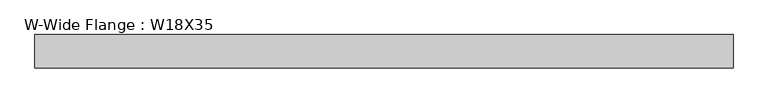
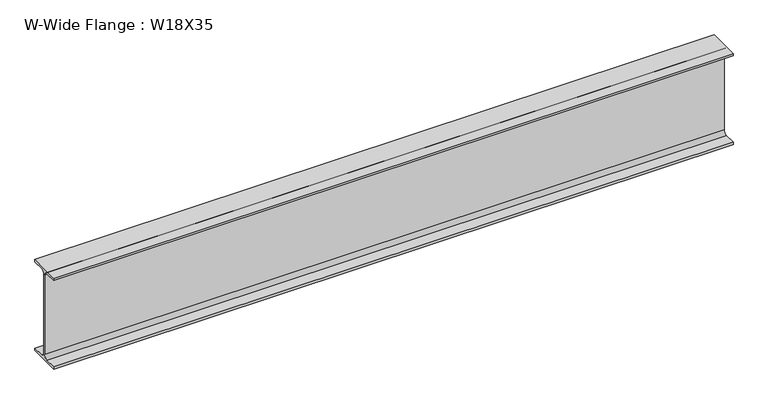
"""IFC4 building model written with IfcOpenShell, lengths in millimetres: beam geometry, W-Wide Flange : W18X35."""

import ifcopenshell
import ifcopenshell.guid

model = None  # the IFC model being written
_history = None  # IfcOwnerHistory: only IFC2X3 demands one
_inside = {}  # id of a spatial element -> (the spatial element, [elements in it])
_under = {}  # id of a project, library or spatial element -> (it, [spatial elements below it])
_declared = {}  # id of a project -> (the project, [libraries it declares])
_typed = {}  # id of a type object -> (the type object, [elements of that type])
_made_of = {}  # id of a material, layer set ... -> (it, [elements and type objects made of it])


def new_model(schema):
    """Start an empty IFC model of exactly this schema.

    Asked for "IFC4X3", IfcOpenShell would pick the latest addendum, in which some entities
    have other attributes; the version numbers below select the first issue.
    IFC2X3 requires an IfcOwnerHistory on every rooted entity: one is made here for all.
    """
    global model, _history
    if schema == "IFC4X3":
        model = ifcopenshell.file(schema_version=(4, 3, 0, 0))
    else:
        model = ifcopenshell.file(schema=schema)
    _inside.clear()
    _under.clear()
    _declared.clear()
    _typed.clear()
    _made_of.clear()
    _history = None
    if model.schema == "IFC2X3":
        org = make("IfcOrganization", Name="unknown")
        user = make(
            "IfcPersonAndOrganization",
            ThePerson=make("IfcPerson", FamilyName="unknown"),
            TheOrganization=org,
        )
        app = make(
            "IfcApplication",
            ApplicationDeveloper=org,
            Version="unknown",
            ApplicationFullName="unknown",
            ApplicationIdentifier="unknown",
        )
        _history = make(
            "IfcOwnerHistory",
            OwningUser=user,
            OwningApplication=app,
            ChangeAction="ADDED",
            CreationDate=0,
        )
    return model


def make(cls, **values):
    """One entity of the class cls with the attributes given. An attribute that is None is left unset."""
    return model.create_entity(
        cls, **{name: value for name, value in values.items() if value is not None}
    )


def rooted(cls, **values):
    """An entity with a GlobalId (a new one), such as an element, a storey or a relation."""
    return make(cls, GlobalId=ifcopenshell.guid.new(), OwnerHistory=_history, **values)


def si_unit(unit_type, name, prefix=None):
    """IfcSIUnit, for example si_unit("LENGTHUNIT", "METRE", prefix="MILLI")."""
    return make("IfcSIUnit", UnitType=unit_type, Prefix=prefix, Name=name)


def assignment(units):
    """IfcUnitAssignment: the units of a project."""
    return None if units is None else make("IfcUnitAssignment", Units=units)


def point(xyz):
    """IfcCartesianPoint."""
    return None if xyz is None else make("IfcCartesianPoint", Coordinates=xyz)


def direction(xyz):
    """IfcDirection."""
    return None if xyz is None else make("IfcDirection", DirectionRatios=xyz)


def frame(location, z_axis=None, x_axis=None):
    """IfcAxis2Placement3D, a coordinate frame: its origin and axes. An axis left out is left unset."""
    return make(
        "IfcAxis2Placement3D",
        Location=point(location),
        Axis=direction(z_axis),
        RefDirection=direction(x_axis),
    )


def frame_2d(location, x_axis=None):
    """IfcAxis2Placement2D, a coordinate frame in the plane: its origin and x axis."""
    return make(
        "IfcAxis2Placement2D", Location=point(location), RefDirection=direction(x_axis)
    )


def origin():
    """The frame at (0, 0, 0) with its axes left unset."""
    return frame((0.0, 0.0, 0.0))


def place(relative_to, where):
    """IfcLocalPlacement: puts the frame where relative to a parent placement (None: the world)."""
    return make(
        "IfcLocalPlacement", PlacementRelTo=relative_to, RelativePlacement=where
    )


def context(
    kind, dimensions, precision=None, world=None, true_north=None, identifier=None
):
    """IfcGeometricRepresentationContext, for example the 3D "Model" context."""
    return make(
        "IfcGeometricRepresentationContext",
        ContextIdentifier=identifier,
        ContextType=kind,
        CoordinateSpaceDimension=dimensions,
        Precision=precision,
        WorldCoordinateSystem=world,
        TrueNorth=true_north,
    )


def project(units=None, contexts=None):
    """IfcProject with its units and contexts."""
    return rooted(
        "IfcProject",
        Name="project",
        RepresentationContexts=contexts,
        UnitsInContext=assignment(units),
    )


def spatial(cls, under=None, at=None, **own):
    """A site, building, storey or space (cls), placed at a placement, below another one or the project."""
    s = rooted(cls, ObjectPlacement=at, **own)
    if under is not None:
        _under.setdefault(under.id(), (under, []))[1].append(s)
    return s


def polyline(points):
    """IfcPolyline through the points."""
    return make("IfcPolyline", Points=[point(p) for p in points])


def circle_curve(where, radius):
    """IfcCircle in the frame where."""
    return make("IfcCircle", Position=where, Radius=radius)


def trimmed(basis, trim1, trim2, sense, master):
    """IfcTrimmedCurve: the piece of a basis curve between two trims."""
    return make(
        "IfcTrimmedCurve",
        BasisCurve=basis,
        Trim1=trim1,
        Trim2=trim2,
        SenseAgreement=sense,
        MasterRepresentation=master,
    )


def segment(curve, same_sense, transition):
    """IfcCompositeCurveSegment."""
    return make(
        "IfcCompositeCurveSegment",
        Transition=transition,
        SameSense=same_sense,
        ParentCurve=curve,
    )


def composite_curve(segments, self_intersect=None):
    """IfcCompositeCurve: segments joined end to end."""
    return make("IfcCompositeCurve", Segments=segments, SelfIntersect=self_intersect)


def outline(outer, holes=None, kind="AREA"):
    """IfcArbitraryClosedProfileDef: a profile drawn as a closed curve; with holes, ...WithVoids."""
    if holes is None:
        return make("IfcArbitraryClosedProfileDef", ProfileType=kind, OuterCurve=outer)
    return make(
        "IfcArbitraryProfileDefWithVoids",
        ProfileType=kind,
        OuterCurve=outer,
        InnerCurves=holes,
    )


def extrude(swept, where, along, depth):
    """IfcExtrudedAreaSolid: the profile swept, set in the frame where, extruded along a direction by depth."""
    return make(
        "IfcExtrudedAreaSolid",
        SweptArea=swept,
        Position=where,
        ExtrudedDirection=direction(along),
        Depth=depth,
    )


def shape(context_of_items, identifier, shape_type, items):
    """IfcShapeRepresentation: the items that make up one representation, for example the "Body"."""
    return make(
        "IfcShapeRepresentation",
        ContextOfItems=context_of_items,
        RepresentationIdentifier=identifier,
        RepresentationType=shape_type,
        Items=items,
    )


def source(mapping_origin, context_of_items, identifier, shape_type, items):
    """IfcRepresentationMap: a shape defined once, which mapped items show again and again."""
    return make(
        "IfcRepresentationMap",
        MappingOrigin=mapping_origin,
        MappedRepresentation=shape(context_of_items, identifier, shape_type, items),
    )


def transform(
    local_origin,
    x_axis=None,
    y_axis=None,
    z_axis=None,
    scale=None,
    scale2=None,
    scale3=None,
    uniform=True,
):
    """IfcCartesianTransformationOperator3D, or its non-uniform kind. x_axis, y_axis, z_axis: its Axis1, 2, 3."""
    if uniform:
        return make(
            "IfcCartesianTransformationOperator3D",
            Axis1=direction(x_axis),
            Axis2=direction(y_axis),
            LocalOrigin=point(local_origin),
            Scale=scale,
            Axis3=direction(z_axis),
        )
    return make(
        "IfcCartesianTransformationOperator3DnonUniform",
        Axis1=direction(x_axis),
        Axis2=direction(y_axis),
        LocalOrigin=point(local_origin),
        Scale=scale,
        Axis3=direction(z_axis),
        Scale2=scale2,
        Scale3=scale3,
    )


def mapped(mapping_source, mapping_target):
    """IfcMappedItem: shows the shape of a source again, moved by a transform."""
    return make(
        "IfcMappedItem", MappingSource=mapping_source, MappingTarget=mapping_target
    )


def made_of(thing, what):
    """Note that an element or type object is made of a material, layer set ...; save() writes the relation."""
    if what is not None:
        _made_of.setdefault(what.id(), (what, []))[1].append(thing)
    return thing


def element(
    cls,
    number,
    at=None,
    inside=None,
    cuts=None,
    type_object=None,
    material=None,
    context=None,
    identifier="Body",
    shape_type=None,
    held_by="IfcProductDefinitionShape",
    body=None,
    shapes=None,
    **own,
):
    """One element of the class cls, such as IfcWall. Its Tag is "e" and its number.

    at: its placement. inside: the storey or other place that contains it. cuts: it is an
    opening in that element (IfcRelVoidsElement). A single representation is given by context,
    identifier, shape_type and body (its items); several are given by shapes. held_by: the class
    of the entity that holds the representations. save() writes the other relations.
    """
    e = rooted(cls, Tag="e%d" % number, ObjectPlacement=at, **own)
    if body is not None:
        shapes = [shape(context, identifier, shape_type, body)]
    if shapes is not None:
        e.Representation = make(held_by, Representations=shapes)
    if inside is not None:
        _inside.setdefault(inside.id(), (inside, []))[1].append(e)
    if cuts is not None:
        rooted(
            "IfcRelVoidsElement", RelatingBuildingElement=cuts, RelatedOpeningElement=e
        )
    if type_object is not None:
        _typed.setdefault(type_object.id(), (type_object, []))[1].append(e)
    return made_of(e, material)


def aggregate(whole, parts):
    """IfcRelAggregates: a whole, such as a stair, and the parts it consists of."""
    return rooted("IfcRelAggregates", RelatingObject=whole, RelatedObjects=parts)


def save(model, path):
    """Write the relations noted so far, then the file.

    IfcRelAggregates (storeys below a building ...), IfcRelContainedInSpatialStructure (elements
    in a storey), IfcRelDefinesByType, IfcRelAssociatesMaterial and IfcRelDeclares: one each for
    every whole, place, type object, material and project.
    """
    for whole, parts in _under.values():
        aggregate(whole, parts)
    for where, things in _inside.values():
        rooted(
            "IfcRelContainedInSpatialStructure",
            RelatedElements=things,
            RelatingStructure=where,
        )
    for kind, things in _typed.values():
        rooted("IfcRelDefinesByType", RelatedObjects=things, RelatingType=kind)
    for what, things in _made_of.values():
        rooted("IfcRelAssociatesMaterial", RelatedObjects=things, RelatingMaterial=what)
    for by, libraries in _declared.values():
        rooted("IfcRelDeclares", RelatingContext=by, RelatedDefinitions=libraries)
    model.write(path)


def w_wide_flange_w18x35_64c4e646(model_context):
    return source(origin(), model_context, "Body", "SweptSolid", [
        extrude(outline(composite_curve([segment(polyline([(76.2, -213.995), (76.2, -224.79), (-76.2, -224.79), (-76.2, -213.995), (-21.59, -213.995)]), True, "CONTINUOUS"), segment(trimmed(circle_curve(frame_2d((-21.59, -196.215)), 17.78), [point((-21.59, -213.995))], [point((-3.81, -196.215))], True, "CARTESIAN"), True, "CONTINUOUS"), segment(polyline([(-3.81, -196.215), (-3.81, 196.215)]), True, "CONTINUOUS"), segment(trimmed(circle_curve(frame_2d((-21.59, 196.215)), 17.78), [point((-3.81, 196.215))], [point((-21.59, 213.995))], True, "CARTESIAN"), True, "CONTINUOUS"), segment(polyline([(-21.59, 213.995), (-76.2, 213.995), (-76.2, 224.79), (76.2, 224.79), (76.2, 213.995), (21.59, 213.995)]), True, "CONTINUOUS"), segment(trimmed(circle_curve(frame_2d((21.59, 196.215)), 17.78), [point((21.59, 213.995))], [point((3.81, 196.215))], True, "CARTESIAN"), True, "CONTINUOUS"), segment(polyline([(3.81, 196.215), (3.81, -196.215)]), True, "CONTINUOUS"), segment(trimmed(circle_curve(frame_2d((21.59, -196.215)), 17.78), [point((3.81, -196.215))], [point((21.59, -213.995))], True, "CARTESIAN"), True, "CONTINUOUS"), segment(polyline([(21.59, -213.995), (76.2, -213.995)]), True, "CONTINUOUS")], self_intersect=False)), frame((-1587.5, 0.0, 0.0), z_axis=(1.0, 0.0, 0.0), x_axis=(0.0, 1.0, 0.0)), (0.0, 0.0, 1.0), 3175.0),
    ])


if __name__ == "__main__":
    model = new_model("IFC4")
    model_context = context("Model", 3, world=origin())
    ifc_project = project(units=[si_unit("LENGTHUNIT", "METRE", prefix="MILLI")], contexts=[model_context])
    site = spatial("IfcSite", under=ifc_project)
    building = spatial("IfcBuilding", under=site)
    placement = place(None, origin())
    w_wide_flange_w18x35_shape = w_wide_flange_w18x35_64c4e646(model_context)
    element("IfcBeam", 1, ObjectType="W-Wide Flange : W18X35", at=placement, inside=building, context=model_context, shape_type="MappedRepresentation", body=[
        mapped(w_wide_flange_w18x35_shape, transform((0.0, 0.0, 0.0), x_axis=(1.0, 0.0, 0.0), y_axis=(0.0, 1.0, 0.0), z_axis=(0.0, 0.0, 1.0))),
    ])
    save(model, "model.ifc")

# Revit data of these elements
# Type "W-Wide Flange : W18X35"
#   Assembly Code = "B10"
#   W = 35
#   Length [instance default] = 5' - 0"
#   bf = 0' - 6"
#   d = 1' - 5.7"
#   k = 0' - 1 1/8"
#   k2 = 0' - 0.7"
#   tf = 0' - 0.425"
#   tw = 0' - 0.3"
#   A = 0.0715278 SF
#   Structural Material [instance default] = Steel ASTM A992
# Element 1 (IfcBeam, "W-Wide Flange : W18X35")
#   Structural Material = Steel ASTM A36
#   Materials on its faces: "Steel ASTM A36"
# Materials
#   "Steel ASTM A992": class "Metal", colour RGB 199 199 199, transparency 0, Description = "Structural steel 50ksi", Cost = 0
#   "Steel ASTM A36": class "Metal", colour RGB 199 199 199, transparency 0, Description = "Structural steel, ASTM A36 Grade B, mill finish", Cost = 0
